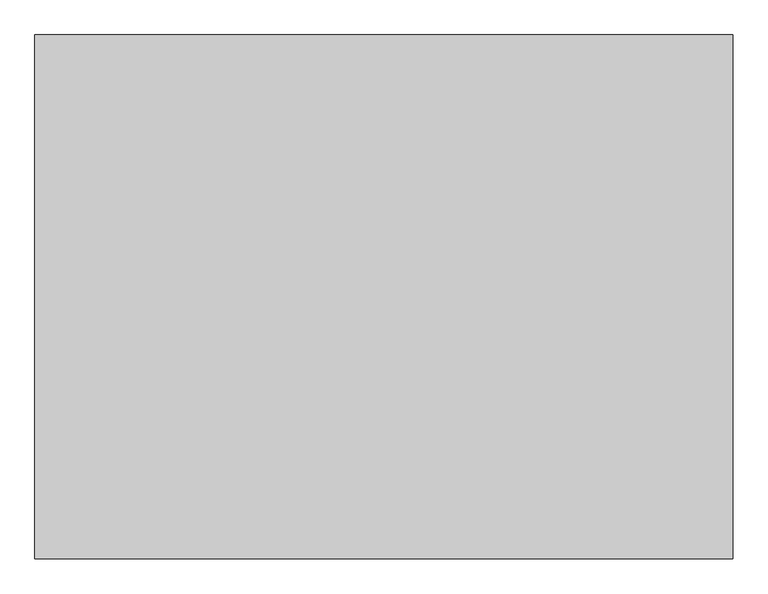
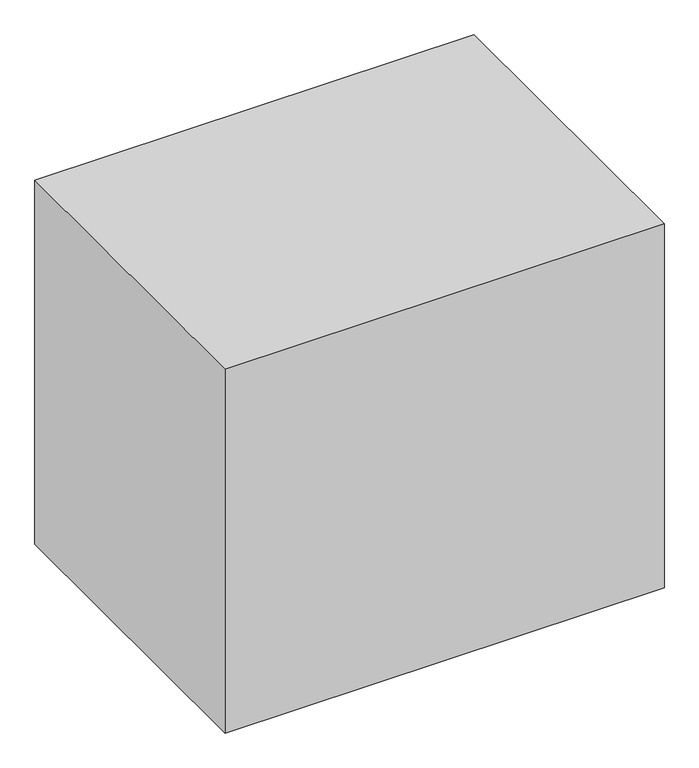
"""IFC4 building model written with IfcOpenShell, lengths in millimetres: proxy geometry, Space Planning Box_hec : Space Planning Box_hec."""

from ifc_helpers import new_model, si_unit, origin, origin_with_axes, place, context, project, spatial, polyline, outline, extrude, source, transform, mapped, element, save


def generic_models_4c644d41(model_context):
    return source(origin(), model_context, "Body", "SweptSolid", [
        extrude(outline(polyline([(2000.0, 1500.0), (2000.0, -1500.0), (-2000.0, -1500.0), (-2000.0, 1500.0), (2000.0, 1500.0)])), origin_with_axes(), (0.0, 0.0, 1.0), 3500.0),
    ])


if __name__ == "__main__":
    model = new_model("IFC4")
    model_context = context("Model", 3, world=origin())
    ifc_project = project(units=[si_unit("LENGTHUNIT", "METRE", prefix="MILLI")], contexts=[model_context])
    site = spatial("IfcSite", under=ifc_project)
    building = spatial("IfcBuilding", under=site)
    placement = place(None, origin())
    generic_models_shape = generic_models_4c644d41(model_context)
    element("IfcBuildingElementProxy", 1, Name="Space Planning Box_hec : Space Planning Box_hec", ObjectType="Space Planning Box_hec : Space Planning Box_hec", at=placement, inside=building, context=model_context, shape_type="MappedRepresentation", body=[
        mapped(generic_models_shape, transform((0.0, 0.0, 0.0), x_axis=(1.0, 0.0, 0.0), y_axis=(0.0, 1.0, 0.0), z_axis=(0.0, 0.0, 1.0))),
    ])
    save(model, "model.ifc")

# Revit data of these elements
# Type "Space Planning Box_hec : Space Planning Box_hec"
#   Type Comments = "..."
#   Room Name [instance default] = "?"
#   Interior Finish [instance default] = ""
#   Exterior Finish [instance default] = ""
#   Department [instance default] = ""
#   Assembly Code = "..."
#   ceiling height [instance default] = 0
#   Width [instance default] = 1524 mm
#   Program Area [instance default] = 0.00 m²
#   Length [instance default] = 1524 mm
#   Height [instance default] = 1524 mm
#   Area [instance default] = 2.32258 m²
#   Fill Color [instance default] = Cyan
#   Default Elevation = 0
# Element 1 (IfcBuildingElementProxy, "Space Planning Box_hec : Space Planning Box_hec")
#   Room Name = "Elevator"
#   Interior Finish = "N/A..N/A..N/A,,N/A..N/A,,,,CL3..N/A"
#   Exterior Finish = "N/A..N/A,,EW2..N/A..N/A"
#   Department = "AR"
#   Width = 4000 mm
#   Length = 3000 mm
#   Height = 3500 mm
#   Area = 12.00 m²
#   Materials on its faces: "Cyan"
# Materials
#   "Cyan": class "Generic", colour RGB 0 255 255, transparency 0.2, Cost = 0
